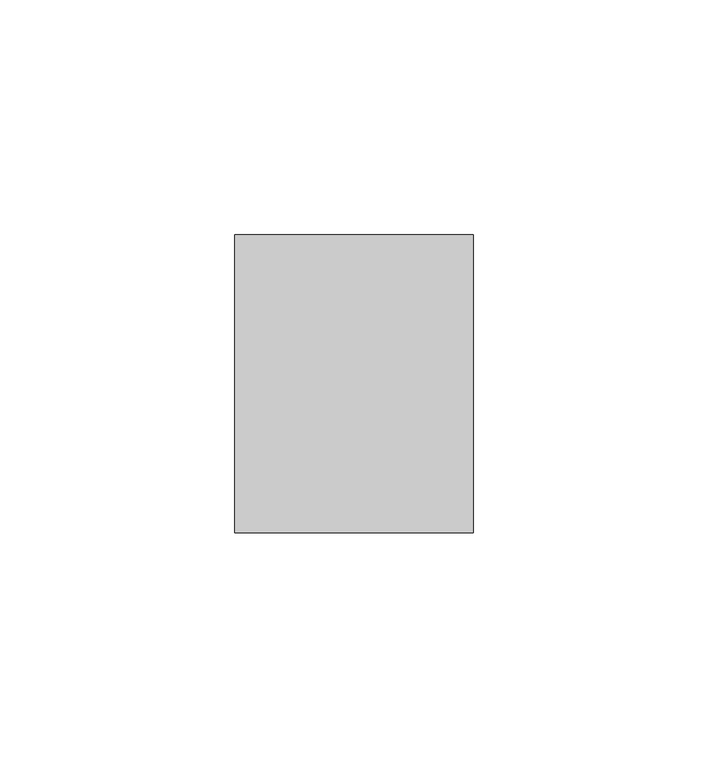
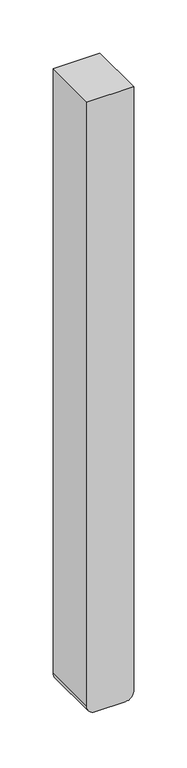
"""IFC4 building model written with IfcOpenShell, lengths in millimetres: proxy geometry, Generic Models 221:Generic Models 219:154171 : Generic Models 221:Generic Models 219:154171."""

import ifcopenshell
import ifcopenshell.guid

model = None  # the IFC model being written
_history = None  # IfcOwnerHistory: only IFC2X3 demands one
_inside = {}  # id of a spatial element -> (the spatial element, [elements in it])
_under = {}  # id of a project, library or spatial element -> (it, [spatial elements below it])
_declared = {}  # id of a project -> (the project, [libraries it declares])
_typed = {}  # id of a type object -> (the type object, [elements of that type])
_made_of = {}  # id of a material, layer set ... -> (it, [elements and type objects made of it])


def new_model(schema):
    """Start an empty IFC model of exactly this schema.

    Asked for "IFC4X3", IfcOpenShell would pick the latest addendum, in which some entities
    have other attributes; the version numbers below select the first issue.
    IFC2X3 requires an IfcOwnerHistory on every rooted entity: one is made here for all.
    """
    global model, _history
    if schema == "IFC4X3":
        model = ifcopenshell.file(schema_version=(4, 3, 0, 0))
    else:
        model = ifcopenshell.file(schema=schema)
    _inside.clear()
    _under.clear()
    _declared.clear()
    _typed.clear()
    _made_of.clear()
    _history = None
    if model.schema == "IFC2X3":
        org = make("IfcOrganization", Name="unknown")
        user = make(
            "IfcPersonAndOrganization",
            ThePerson=make("IfcPerson", FamilyName="unknown"),
            TheOrganization=org,
        )
        app = make(
            "IfcApplication",
            ApplicationDeveloper=org,
            Version="unknown",
            ApplicationFullName="unknown",
            ApplicationIdentifier="unknown",
        )
        _history = make(
            "IfcOwnerHistory",
            OwningUser=user,
            OwningApplication=app,
            ChangeAction="ADDED",
            CreationDate=0,
        )
    return model


def make(cls, **values):
    """One entity of the class cls with the attributes given. An attribute that is None is left unset."""
    return model.create_entity(
        cls, **{name: value for name, value in values.items() if value is not None}
    )


def rooted(cls, **values):
    """An entity with a GlobalId (a new one), such as an element, a storey or a relation."""
    return make(cls, GlobalId=ifcopenshell.guid.new(), OwnerHistory=_history, **values)


def si_unit(unit_type, name, prefix=None):
    """IfcSIUnit, for example si_unit("LENGTHUNIT", "METRE", prefix="MILLI")."""
    return make("IfcSIUnit", UnitType=unit_type, Prefix=prefix, Name=name)


def assignment(units):
    """IfcUnitAssignment: the units of a project."""
    return None if units is None else make("IfcUnitAssignment", Units=units)


def point(xyz):
    """IfcCartesianPoint."""
    return None if xyz is None else make("IfcCartesianPoint", Coordinates=xyz)


def direction(xyz):
    """IfcDirection."""
    return None if xyz is None else make("IfcDirection", DirectionRatios=xyz)


def frame(location, z_axis=None, x_axis=None):
    """IfcAxis2Placement3D, a coordinate frame: its origin and axes. An axis left out is left unset."""
    return make(
        "IfcAxis2Placement3D",
        Location=point(location),
        Axis=direction(z_axis),
        RefDirection=direction(x_axis),
    )


def frame_2d(location, x_axis=None):
    """IfcAxis2Placement2D, a coordinate frame in the plane: its origin and x axis."""
    return make(
        "IfcAxis2Placement2D", Location=point(location), RefDirection=direction(x_axis)
    )


def origin():
    """The frame at (0, 0, 0) with its axes left unset."""
    return frame((0.0, 0.0, 0.0))


def place(relative_to, where):
    """IfcLocalPlacement: puts the frame where relative to a parent placement (None: the world)."""
    return make(
        "IfcLocalPlacement", PlacementRelTo=relative_to, RelativePlacement=where
    )


def context(
    kind, dimensions, precision=None, world=None, true_north=None, identifier=None
):
    """IfcGeometricRepresentationContext, for example the 3D "Model" context."""
    return make(
        "IfcGeometricRepresentationContext",
        ContextIdentifier=identifier,
        ContextType=kind,
        CoordinateSpaceDimension=dimensions,
        Precision=precision,
        WorldCoordinateSystem=world,
        TrueNorth=true_north,
    )


def project(units=None, contexts=None):
    """IfcProject with its units and contexts."""
    return rooted(
        "IfcProject",
        Name="project",
        RepresentationContexts=contexts,
        UnitsInContext=assignment(units),
    )


def spatial(cls, under=None, at=None, **own):
    """A site, building, storey or space (cls), placed at a placement, below another one or the project."""
    s = rooted(cls, ObjectPlacement=at, **own)
    if under is not None:
        _under.setdefault(under.id(), (under, []))[1].append(s)
    return s


def polyline(points):
    """IfcPolyline through the points."""
    return make("IfcPolyline", Points=[point(p) for p in points])


def circle_curve(where, radius):
    """IfcCircle in the frame where."""
    return make("IfcCircle", Position=where, Radius=radius)


def trimmed(basis, trim1, trim2, sense, master):
    """IfcTrimmedCurve: the piece of a basis curve between two trims."""
    return make(
        "IfcTrimmedCurve",
        BasisCurve=basis,
        Trim1=trim1,
        Trim2=trim2,
        SenseAgreement=sense,
        MasterRepresentation=master,
    )


def segment(curve, same_sense, transition):
    """IfcCompositeCurveSegment."""
    return make(
        "IfcCompositeCurveSegment",
        Transition=transition,
        SameSense=same_sense,
        ParentCurve=curve,
    )


def composite_curve(segments, self_intersect=None):
    """IfcCompositeCurve: segments joined end to end."""
    return make("IfcCompositeCurve", Segments=segments, SelfIntersect=self_intersect)


def outline(outer, holes=None, kind="AREA"):
    """IfcArbitraryClosedProfileDef: a profile drawn as a closed curve; with holes, ...WithVoids."""
    if holes is None:
        return make("IfcArbitraryClosedProfileDef", ProfileType=kind, OuterCurve=outer)
    return make(
        "IfcArbitraryProfileDefWithVoids",
        ProfileType=kind,
        OuterCurve=outer,
        InnerCurves=holes,
    )


def extrude(swept, where, along, depth):
    """IfcExtrudedAreaSolid: the profile swept, set in the frame where, extruded along a direction by depth."""
    return make(
        "IfcExtrudedAreaSolid",
        SweptArea=swept,
        Position=where,
        ExtrudedDirection=direction(along),
        Depth=depth,
    )


def shape(context_of_items, identifier, shape_type, items):
    """IfcShapeRepresentation: the items that make up one representation, for example the "Body"."""
    return make(
        "IfcShapeRepresentation",
        ContextOfItems=context_of_items,
        RepresentationIdentifier=identifier,
        RepresentationType=shape_type,
        Items=items,
    )


def source(mapping_origin, context_of_items, identifier, shape_type, items):
    """IfcRepresentationMap: a shape defined once, which mapped items show again and again."""
    return make(
        "IfcRepresentationMap",
        MappingOrigin=mapping_origin,
        MappedRepresentation=shape(context_of_items, identifier, shape_type, items),
    )


def transform(
    local_origin,
    x_axis=None,
    y_axis=None,
    z_axis=None,
    scale=None,
    scale2=None,
    scale3=None,
    uniform=True,
):
    """IfcCartesianTransformationOperator3D, or its non-uniform kind. x_axis, y_axis, z_axis: its Axis1, 2, 3."""
    if uniform:
        return make(
            "IfcCartesianTransformationOperator3D",
            Axis1=direction(x_axis),
            Axis2=direction(y_axis),
            LocalOrigin=point(local_origin),
            Scale=scale,
            Axis3=direction(z_axis),
        )
    return make(
        "IfcCartesianTransformationOperator3DnonUniform",
        Axis1=direction(x_axis),
        Axis2=direction(y_axis),
        LocalOrigin=point(local_origin),
        Scale=scale,
        Axis3=direction(z_axis),
        Scale2=scale2,
        Scale3=scale3,
    )


def mapped(mapping_source, mapping_target):
    """IfcMappedItem: shows the shape of a source again, moved by a transform."""
    return make(
        "IfcMappedItem", MappingSource=mapping_source, MappingTarget=mapping_target
    )


def made_of(thing, what):
    """Note that an element or type object is made of a material, layer set ...; save() writes the relation."""
    if what is not None:
        _made_of.setdefault(what.id(), (what, []))[1].append(thing)
    return thing


def element(
    cls,
    number,
    at=None,
    inside=None,
    cuts=None,
    type_object=None,
    material=None,
    context=None,
    identifier="Body",
    shape_type=None,
    held_by="IfcProductDefinitionShape",
    body=None,
    shapes=None,
    **own,
):
    """One element of the class cls, such as IfcWall. Its Tag is "e" and its number.

    at: its placement. inside: the storey or other place that contains it. cuts: it is an
    opening in that element (IfcRelVoidsElement). A single representation is given by context,
    identifier, shape_type and body (its items); several are given by shapes. held_by: the class
    of the entity that holds the representations. save() writes the other relations.
    """
    e = rooted(cls, Tag="e%d" % number, ObjectPlacement=at, **own)
    if body is not None:
        shapes = [shape(context, identifier, shape_type, body)]
    if shapes is not None:
        e.Representation = make(held_by, Representations=shapes)
    if inside is not None:
        _inside.setdefault(inside.id(), (inside, []))[1].append(e)
    if cuts is not None:
        rooted(
            "IfcRelVoidsElement", RelatingBuildingElement=cuts, RelatedOpeningElement=e
        )
    if type_object is not None:
        _typed.setdefault(type_object.id(), (type_object, []))[1].append(e)
    return made_of(e, material)


def aggregate(whole, parts):
    """IfcRelAggregates: a whole, such as a stair, and the parts it consists of."""
    return rooted("IfcRelAggregates", RelatingObject=whole, RelatedObjects=parts)


def save(model, path):
    """Write the relations noted so far, then the file.

    IfcRelAggregates (storeys below a building ...), IfcRelContainedInSpatialStructure (elements
    in a storey), IfcRelDefinesByType, IfcRelAssociatesMaterial and IfcRelDeclares: one each for
    every whole, place, type object, material and project.
    """
    for whole, parts in _under.values():
        aggregate(whole, parts)
    for where, things in _inside.values():
        rooted(
            "IfcRelContainedInSpatialStructure",
            RelatedElements=things,
            RelatingStructure=where,
        )
    for kind, things in _typed.values():
        rooted("IfcRelDefinesByType", RelatedObjects=things, RelatingType=kind)
    for what, things in _made_of.values():
        rooted("IfcRelAssociatesMaterial", RelatedObjects=things, RelatingMaterial=what)
    for by, libraries in _declared.values():
        rooted("IfcRelDeclares", RelatingContext=by, RelatedDefinitions=libraries)
    model.write(path)


def generic_models_70cb40c6(model_context):
    return source(origin(), model_context, "Body", "SweptSolid", [
        extrude(outline(composite_curve([segment(polyline([(1263.764977, 7788.153213), (568.1395172, 7788.153213)]), True, "CONTINUOUS"), segment(trimmed(circle_curve(frame_2d((568.1395172, 7796.992413)), 8.8392), [point((568.1395172, 7788.153213))], [point((559.3003172, 7796.992413))], False, "CARTESIAN"), True, "CONTINUOUS"), segment(polyline([(559.3003172, 7796.992413), (559.3003172, 7830.114013)]), True, "CONTINUOUS"), segment(trimmed(circle_curve(frame_2d((568.1395172, 7830.114013)), 8.8392), [point((559.3003172, 7830.114013))], [point((568.1395172, 7838.953213))], False, "CARTESIAN"), True, "CONTINUOUS"), segment(polyline([(568.1395172, 7838.953213), (1263.764977, 7838.953213), (1263.764977, 7788.153213)]), True, "CONTINUOUS")], self_intersect=False)), frame((0.0, 4691.511949, 0.0), z_axis=(0.0, 1.0, 0.0), x_axis=(0.0, 0.0, 1.0)), (0.0, 0.0, 1.0), 63.500874),
    ])


if __name__ == "__main__":
    model = new_model("IFC4")
    model_context = context("Model", 3, world=origin())
    ifc_project = project(units=[si_unit("LENGTHUNIT", "METRE", prefix="MILLI")], contexts=[model_context])
    site = spatial("IfcSite", under=ifc_project)
    building = spatial("IfcBuilding", under=site)
    placement = place(None, origin())
    generic_models_shape = generic_models_70cb40c6(model_context)
    element("IfcBuildingElementProxy", 1, Name="Generic Models 221:Generic Models 219:154171 : Generic Models 221:Generic Models 219:154171", ObjectType="Generic Models 221:Generic Models 219:154171 : Generic Models 221:Generic Models 219:154171", at=placement, inside=building, context=model_context, shape_type="MappedRepresentation", body=[
        mapped(generic_models_shape, transform((0.0, 0.0, 0.0), x_axis=(1.0, 0.0, 0.0), y_axis=(0.0, 1.0, 0.0), z_axis=(0.0, 0.0, 1.0))),
    ])
    save(model, "model.ifc")

# Revit data of these elements
# Type "Generic Models 221:Generic Models 219:154171 : Generic Models 221:Generic Models 219:154171"
#   NameOverride = "Generic Models 221:Generic Models 219:154171"
#   ObjectTypeOverride = "Generic Models 221:Generic Models 219"
#   Reference = "Generic Models 219"
#   Category = "Generic Models"
#   Tag = "154171"
# Element 1 (IfcBuildingElementProxy, "Generic Models 221:Generic Models 219:154171 : Generic Models 221:Generic Models 219:154171")
#   Materials on its faces: "_2x3 STEEL PROFILE - METALIZED, PRIMED & PAINTED (COLOR PER ARCHITECT)"
# Materials
#   "_2x3 STEEL PROFILE - METALIZED, PRIMED & PAINTED (COLOR PER ARCHITECT)": class "Metal", colour RGB 199 199 199, transparency 0, Description = "Structural steel 50ksi", Cost = 0
